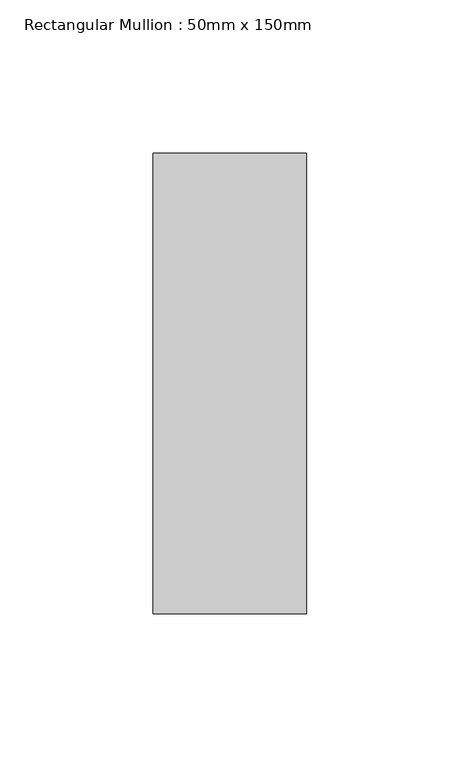
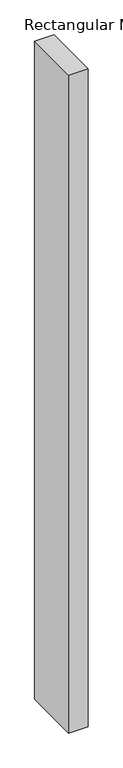
"""IFC4 building model written with IfcOpenShell, lengths in millimetres: member geometry, Rectangular Mullion : 50mm x 150mm."""

from ifc_helpers import new_model, si_unit, frame, origin, place, context, project, spatial, polyline, outline, extrude, source, transform, mapped, element, save


def rectangular_mullion_50mm_x_150mm_0af69dda(model_context):
    return source(origin(), model_context, "Body", "SweptSolid", [
        extrude(outline(polyline([(25.0, 75.0), (25.0, -75.0), (-25.0, -75.0), (-25.0, 75.0), (25.0, 75.0)])), frame((0.0, 0.0, -1780.0000003), z_axis=(0.0, 0.0, 1.0), x_axis=(1.0, 0.0, 0.0)), (0.0, 0.0, 1.0), 1780.0000003),
    ])


if __name__ == "__main__":
    model = new_model("IFC4")
    model_context = context("Model", 3, world=origin())
    ifc_project = project(units=[si_unit("LENGTHUNIT", "METRE", prefix="MILLI")], contexts=[model_context])
    site = spatial("IfcSite", under=ifc_project)
    building = spatial("IfcBuilding", under=site)
    placement = place(None, origin())
    rectangular_mullion_50mm_x_150mm_shape = rectangular_mullion_50mm_x_150mm_0af69dda(model_context)
    element("IfcMember", 1, ObjectType="Rectangular Mullion : 50mm x 150mm", at=placement, inside=building, context=model_context, shape_type="MappedRepresentation", body=[
        mapped(rectangular_mullion_50mm_x_150mm_shape, transform((0.0, 0.0, 0.0), x_axis=(1.0, 0.0, 0.0), y_axis=(0.0, 1.0, 0.0), z_axis=(0.0, 0.0, 1.0))),
    ])
    save(model, "model.ifc")

# Revit data of these elements
# Type "Rectangular Mullion : 50mm x 150mm"
#   built-in parameter 1007304 = 0.492126 (stored number, unit not read)
#   built-in parameter 1007301 = 0.082021 (stored number, unit not read)
#   built-in parameter 1007300 = 0.082021 (stored number, unit not read)
# Element 1 (IfcMember, "Rectangular Mullion : 50mm x 150mm")
#   Materials on its faces: "Aluminum"
# Materials
#   "Aluminum": class "Metal", colour RGB 244 244 244, transparency 0, Description = "Aluminum 6061", Cost = 0
